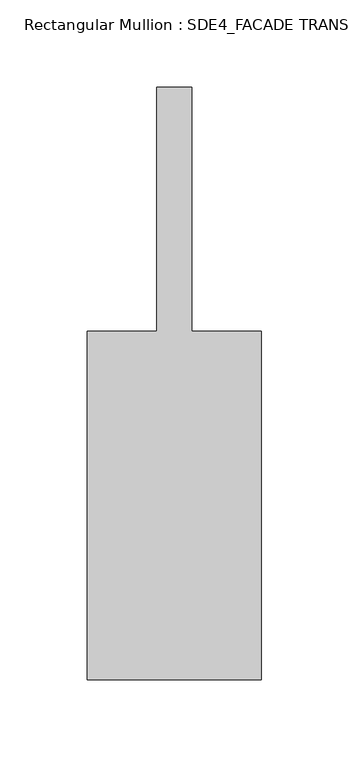
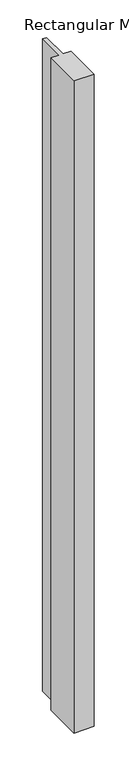
"""IFC4 building model written with IfcOpenShell, lengths in millimetres: member geometry, Rectangular Mullion : SDE4_FACADE TRANSOM TYPE 1."""

from ifc_helpers import new_model, si_unit, frame, origin, place, context, project, spatial, polyline, outline, extrude, source, transform, mapped, element, save


def rectangular_mullion_sde4_facade_transom_type_1_af42bee6(model_context):
    return source(origin(), model_context, "Body", "SweptSolid", [
        extrude(outline(polyline([(50.0, -132.5), (-50.0, -132.5), (-50.0, 67.5), (-10.0, 67.5), (-10.0, 207.5), (10.0, 207.5), (10.0, 67.5), (50.0, 67.5), (50.0, -132.5)])), frame((0.0, 0.0, -3439.0), z_axis=(0.0, 0.0, 1.0), x_axis=(1.0, 0.0, 0.0)), (0.0, 0.0, 1.0), 3439.0),
    ])


if __name__ == "__main__":
    model = new_model("IFC4")
    model_context = context("Model", 3, world=origin())
    ifc_project = project(units=[si_unit("LENGTHUNIT", "METRE", prefix="MILLI")], contexts=[model_context])
    site = spatial("IfcSite", under=ifc_project)
    building = spatial("IfcBuilding", under=site)
    placement = place(None, origin())
    rectangular_mullion_sde4_facade_transom_type_1_shape = rectangular_mullion_sde4_facade_transom_type_1_af42bee6(model_context)
    element("IfcMember", 1, ObjectType="Rectangular Mullion : SDE4_FACADE TRANSOM TYPE 1", at=placement, inside=building, context=model_context, shape_type="MappedRepresentation", body=[
        mapped(rectangular_mullion_sde4_facade_transom_type_1_shape, transform((0.0, 0.0, 0.0), x_axis=(1.0, 0.0, 0.0), y_axis=(0.0, 1.0, 0.0), z_axis=(0.0, 0.0, 1.0))),
    ])
    save(model, "model.ifc")

# Revit data of these elements
# Type "Rectangular Mullion : SDE4_FACADE TRANSOM TYPE 1"
#   built-in parameter 1007322 = 1.11549 (stored number, unit not read)
#   built-in parameter 1007321 = 0.164042 (stored number, unit not read)
#   built-in parameter 1007320 = 0.164042 (stored number, unit not read)
